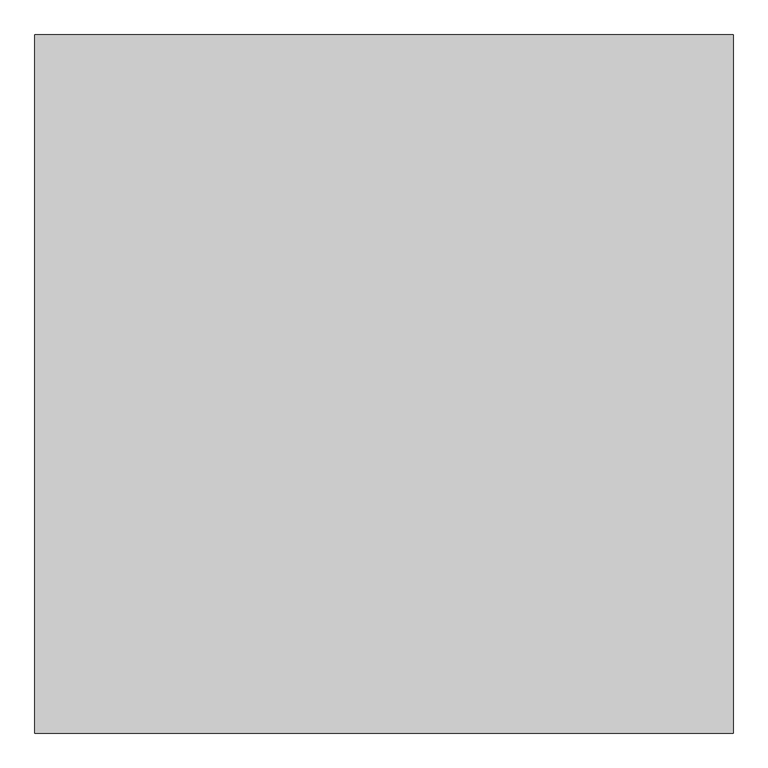
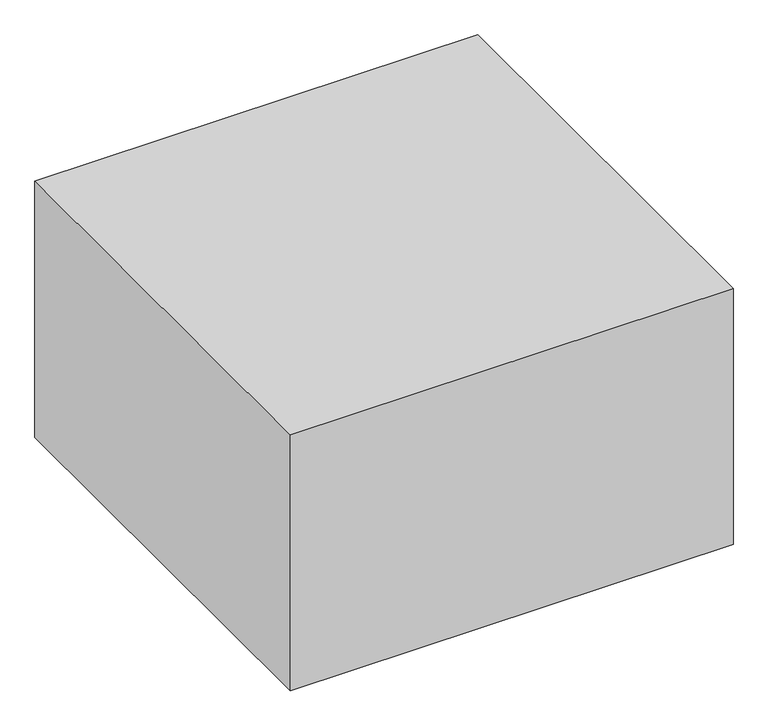
"""IFC4 building model written with IfcOpenShell, lengths in millimetres: proxy geometry, Space Planning Box_hec : Space Planning Box_hec."""

from ifc_helpers import new_model, si_unit, origin, origin_with_axes, place, context, project, spatial, polyline, outline, extrude, source, transform, mapped, element, save


def generic_models_c4e3d020(model_context):
    return source(origin(), model_context, "Body", "SweptSolid", [
        extrude(outline(polyline([(4250.0, 4250.0), (4250.0, -4250.0), (-4250.0, -4250.0), (-4250.0, 4250.0), (4250.0, 4250.0)])), origin_with_axes(), (0.0, 0.0, 1.0), 5200.0),
    ])


if __name__ == "__main__":
    model = new_model("IFC4")
    model_context = context("Model", 3, world=origin())
    ifc_project = project(units=[si_unit("LENGTHUNIT", "METRE", prefix="MILLI")], contexts=[model_context])
    site = spatial("IfcSite", under=ifc_project)
    building = spatial("IfcBuilding", under=site)
    placement = place(None, origin())
    generic_models_shape = generic_models_c4e3d020(model_context)
    element("IfcBuildingElementProxy", 1, Name="Space Planning Box_hec : Space Planning Box_hec", ObjectType="Space Planning Box_hec : Space Planning Box_hec", at=placement, inside=building, context=model_context, shape_type="MappedRepresentation", body=[
        mapped(generic_models_shape, transform((0.0, 0.0, 0.0), x_axis=(1.0, 0.0, 0.0), y_axis=(0.0, 1.0, 0.0), z_axis=(0.0, 0.0, 1.0))),
    ])
    save(model, "model.ifc")

# Revit data of these elements
# Type "Space Planning Box_hec : Space Planning Box_hec"
#   Type Comments = "..."
#   Room Name [instance default] = "?"
#   Interior Finish [instance default] = ""
#   Exterior Finish [instance default] = ""
#   Department [instance default] = ""
#   Assembly Code = "..."
#   ceiling height [instance default] = 0
#   Width [instance default] = 1524 mm
#   Program Area [instance default] = 0.00 m²
#   Length [instance default] = 1524 mm
#   Height [instance default] = 1524 mm
#   Area [instance default] = 2.32258 m²
#   Fill Color [instance default] = Cyan
#   Default Elevation = 0
# Element 1 (IfcBuildingElementProxy, "Space Planning Box_hec : Space Planning Box_hec")
#   Room Name = "Computer Room"
#   Interior Finish = "IW1..N/A,,WB2..N/A,,FL7..N/A,,CL4..N/A"
#   Exterior Finish = "N/A..N/A,,EW1..N/A"
#   Department = "CI"
#   ceiling height = 2700
#   Width = 8500 mm
#   Program Area = 72.25 m²
#   Length = 8500 mm
#   Height = 5200 mm
#   Area = 72.25 m²
#   Fill Color = Yellow
#   Materials on its faces: "Yellow"
# Materials
#   "Cyan": class "Generic", colour RGB 0 255 255, transparency 0.2, Cost = 0
#   "Yellow": class "Generic", colour RGB 255 255 0, transparency 0.2, Cost = 0
